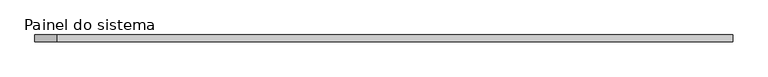
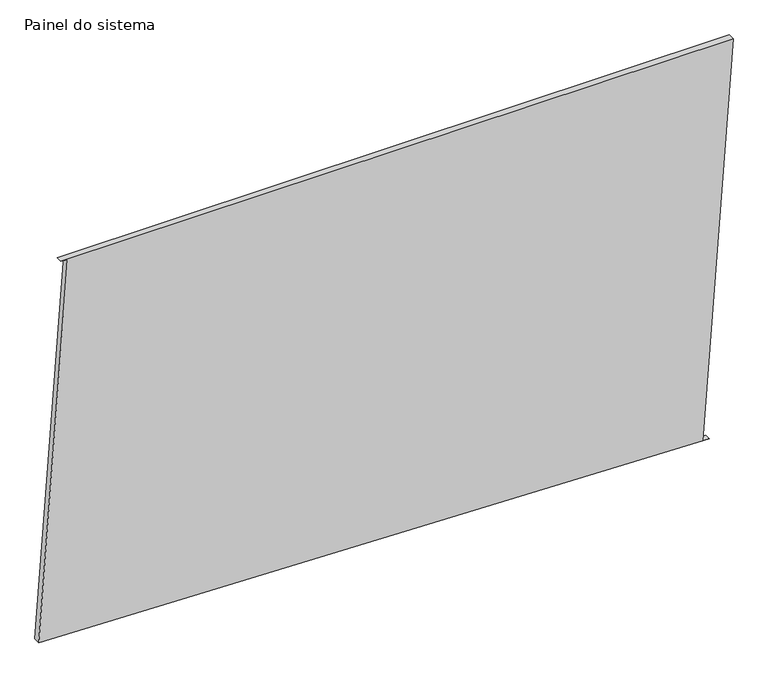
"""IFC4 building model written with IfcOpenShell, lengths in millimetres: plate geometry, Painel do sistema : Envidraçado."""

from ifc_helpers import new_model, si_unit, frame, origin, place, context, project, spatial, polyline, outline, extrude, source, transform, mapped, element, save


def painel_do_sistema_d1c14ea8(model_context):
    return source(origin(), model_context, "Body", "SweptSolid", [
        extrude(outline(polyline([(0.0, 1229.640929), (1.8159485, 1204.7069696), (1576.4565206, 1319.3885618), (1576.4565206, -1234.9880795), (1574.6405721, -1210.0541201), (73.4192812, -1319.3885618), (0.0, 1229.640929)])), frame((0.0, 24.5, 0.0), z_axis=(0.0, 1.0, 0.0), x_axis=(0.0, 0.0, 1.0)), (0.0, 0.0, 1.0), 25.0),
    ])


if __name__ == "__main__":
    model = new_model("IFC4")
    model_context = context("Model", 3, world=origin())
    ifc_project = project(units=[si_unit("LENGTHUNIT", "METRE", prefix="MILLI")], contexts=[model_context])
    site = spatial("IfcSite", under=ifc_project)
    building = spatial("IfcBuilding", under=site)
    placement = place(None, origin())
    painel_do_sistema_shape = painel_do_sistema_d1c14ea8(model_context)
    element("IfcPlate", 1, ObjectType="Painel do sistema : Envidraçado", at=placement, inside=building, context=model_context, shape_type="MappedRepresentation", body=[
        mapped(painel_do_sistema_shape, transform((0.0, 0.0, 0.0), x_axis=(1.0, 0.0, 0.0), y_axis=(0.0, 1.0, 0.0), z_axis=(0.0, 0.0, 1.0))),
    ])
    save(model, "model.ifc")

# Revit data of these elements
# Type "Painel do sistema : Envidraçado"
#   Construction Type Id = "GSP4R"
#   Analytic Construction = "Vidraça única Pilkington 1/8 pol"
#   Visual Light Transmittance = 0.9
#   Solar Heat Gain Coefficient = 0.86
#   Heat Transfer Coefficient (U) = 6.7069 W/(m²·K)
# Element 1 (IfcPlate, "Painel do sistema : Envidraçado")
#   Materials on its faces: "Vidro"
# Materials
#   "Vidro": class "Vidro", colour RGB 0 128 192, transparency 0.9, Description = "Vidro de sílica", Cost = 0
